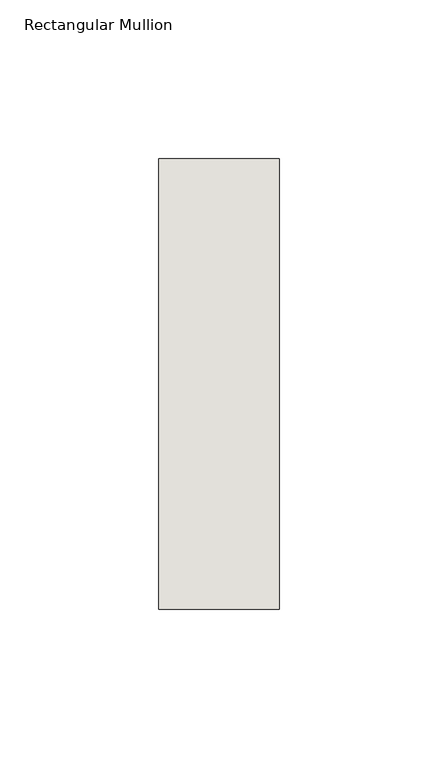
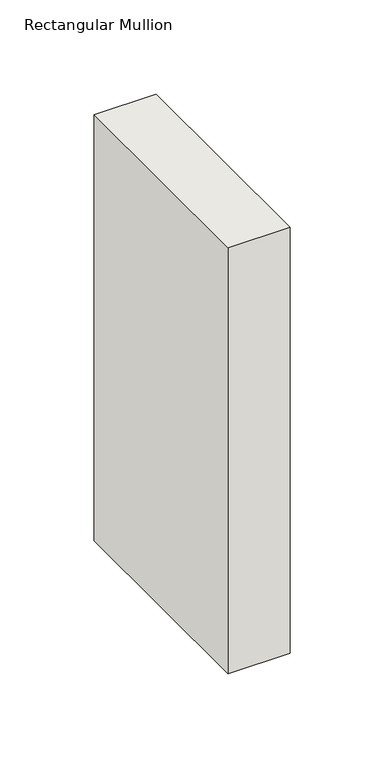
"""IFC4 building model written with IfcOpenShell, lengths in millimetres: wall geometry, Rectangular Mullion : NLRS_21_CWM_hsb-regel 38x142_gen_rsf."""

import ifcopenshell
import ifcopenshell.guid

model = None  # the IFC model being written
_history = None  # IfcOwnerHistory: only IFC2X3 demands one
_inside = {}  # id of a spatial element -> (the spatial element, [elements in it])
_under = {}  # id of a project, library or spatial element -> (it, [spatial elements below it])
_declared = {}  # id of a project -> (the project, [libraries it declares])
_typed = {}  # id of a type object -> (the type object, [elements of that type])
_made_of = {}  # id of a material, layer set ... -> (it, [elements and type objects made of it])


def new_model(schema):
    """Start an empty IFC model of exactly this schema.

    Asked for "IFC4X3", IfcOpenShell would pick the latest addendum, in which some entities
    have other attributes; the version numbers below select the first issue.
    IFC2X3 requires an IfcOwnerHistory on every rooted entity: one is made here for all.
    """
    global model, _history
    if schema == "IFC4X3":
        model = ifcopenshell.file(schema_version=(4, 3, 0, 0))
    else:
        model = ifcopenshell.file(schema=schema)
    _inside.clear()
    _under.clear()
    _declared.clear()
    _typed.clear()
    _made_of.clear()
    _history = None
    if model.schema == "IFC2X3":
        org = make("IfcOrganization", Name="unknown")
        user = make(
            "IfcPersonAndOrganization",
            ThePerson=make("IfcPerson", FamilyName="unknown"),
            TheOrganization=org,
        )
        app = make(
            "IfcApplication",
            ApplicationDeveloper=org,
            Version="unknown",
            ApplicationFullName="unknown",
            ApplicationIdentifier="unknown",
        )
        _history = make(
            "IfcOwnerHistory",
            OwningUser=user,
            OwningApplication=app,
            ChangeAction="ADDED",
            CreationDate=0,
        )
    return model


def make(cls, **values):
    """One entity of the class cls with the attributes given. An attribute that is None is left unset."""
    return model.create_entity(
        cls, **{name: value for name, value in values.items() if value is not None}
    )


def rooted(cls, **values):
    """An entity with a GlobalId (a new one), such as an element, a storey or a relation."""
    return make(cls, GlobalId=ifcopenshell.guid.new(), OwnerHistory=_history, **values)


def si_unit(unit_type, name, prefix=None):
    """IfcSIUnit, for example si_unit("LENGTHUNIT", "METRE", prefix="MILLI")."""
    return make("IfcSIUnit", UnitType=unit_type, Prefix=prefix, Name=name)


def assignment(units):
    """IfcUnitAssignment: the units of a project."""
    return None if units is None else make("IfcUnitAssignment", Units=units)


def point(xyz):
    """IfcCartesianPoint."""
    return None if xyz is None else make("IfcCartesianPoint", Coordinates=xyz)


def direction(xyz):
    """IfcDirection."""
    return None if xyz is None else make("IfcDirection", DirectionRatios=xyz)


def frame(location, z_axis=None, x_axis=None):
    """IfcAxis2Placement3D, a coordinate frame: its origin and axes. An axis left out is left unset."""
    return make(
        "IfcAxis2Placement3D",
        Location=point(location),
        Axis=direction(z_axis),
        RefDirection=direction(x_axis),
    )


def origin():
    """The frame at (0, 0, 0) with its axes left unset."""
    return frame((0.0, 0.0, 0.0))


def place(relative_to, where):
    """IfcLocalPlacement: puts the frame where relative to a parent placement (None: the world)."""
    return make(
        "IfcLocalPlacement", PlacementRelTo=relative_to, RelativePlacement=where
    )


def context(
    kind, dimensions, precision=None, world=None, true_north=None, identifier=None
):
    """IfcGeometricRepresentationContext, for example the 3D "Model" context."""
    return make(
        "IfcGeometricRepresentationContext",
        ContextIdentifier=identifier,
        ContextType=kind,
        CoordinateSpaceDimension=dimensions,
        Precision=precision,
        WorldCoordinateSystem=world,
        TrueNorth=true_north,
    )


def project(units=None, contexts=None):
    """IfcProject with its units and contexts."""
    return rooted(
        "IfcProject",
        Name="project",
        RepresentationContexts=contexts,
        UnitsInContext=assignment(units),
    )


def spatial(cls, under=None, at=None, **own):
    """A site, building, storey or space (cls), placed at a placement, below another one or the project."""
    s = rooted(cls, ObjectPlacement=at, **own)
    if under is not None:
        _under.setdefault(under.id(), (under, []))[1].append(s)
    return s


def polyline(points):
    """IfcPolyline through the points."""
    return make("IfcPolyline", Points=[point(p) for p in points])


def outline(outer, holes=None, kind="AREA"):
    """IfcArbitraryClosedProfileDef: a profile drawn as a closed curve; with holes, ...WithVoids."""
    if holes is None:
        return make("IfcArbitraryClosedProfileDef", ProfileType=kind, OuterCurve=outer)
    return make(
        "IfcArbitraryProfileDefWithVoids",
        ProfileType=kind,
        OuterCurve=outer,
        InnerCurves=holes,
    )


def extrude(swept, where, along, depth):
    """IfcExtrudedAreaSolid: the profile swept, set in the frame where, extruded along a direction by depth."""
    return make(
        "IfcExtrudedAreaSolid",
        SweptArea=swept,
        Position=where,
        ExtrudedDirection=direction(along),
        Depth=depth,
    )


def shape(context_of_items, identifier, shape_type, items):
    """IfcShapeRepresentation: the items that make up one representation, for example the "Body"."""
    return make(
        "IfcShapeRepresentation",
        ContextOfItems=context_of_items,
        RepresentationIdentifier=identifier,
        RepresentationType=shape_type,
        Items=items,
    )


def source(mapping_origin, context_of_items, identifier, shape_type, items):
    """IfcRepresentationMap: a shape defined once, which mapped items show again and again."""
    return make(
        "IfcRepresentationMap",
        MappingOrigin=mapping_origin,
        MappedRepresentation=shape(context_of_items, identifier, shape_type, items),
    )


def transform(
    local_origin,
    x_axis=None,
    y_axis=None,
    z_axis=None,
    scale=None,
    scale2=None,
    scale3=None,
    uniform=True,
):
    """IfcCartesianTransformationOperator3D, or its non-uniform kind. x_axis, y_axis, z_axis: its Axis1, 2, 3."""
    if uniform:
        return make(
            "IfcCartesianTransformationOperator3D",
            Axis1=direction(x_axis),
            Axis2=direction(y_axis),
            LocalOrigin=point(local_origin),
            Scale=scale,
            Axis3=direction(z_axis),
        )
    return make(
        "IfcCartesianTransformationOperator3DnonUniform",
        Axis1=direction(x_axis),
        Axis2=direction(y_axis),
        LocalOrigin=point(local_origin),
        Scale=scale,
        Axis3=direction(z_axis),
        Scale2=scale2,
        Scale3=scale3,
    )


def mapped(mapping_source, mapping_target):
    """IfcMappedItem: shows the shape of a source again, moved by a transform."""
    return make(
        "IfcMappedItem", MappingSource=mapping_source, MappingTarget=mapping_target
    )


def made_of(thing, what):
    """Note that an element or type object is made of a material, layer set ...; save() writes the relation."""
    if what is not None:
        _made_of.setdefault(what.id(), (what, []))[1].append(thing)
    return thing


def element(
    cls,
    number,
    at=None,
    inside=None,
    cuts=None,
    type_object=None,
    material=None,
    context=None,
    identifier="Body",
    shape_type=None,
    held_by="IfcProductDefinitionShape",
    body=None,
    shapes=None,
    **own,
):
    """One element of the class cls, such as IfcWall. Its Tag is "e" and its number.

    at: its placement. inside: the storey or other place that contains it. cuts: it is an
    opening in that element (IfcRelVoidsElement). A single representation is given by context,
    identifier, shape_type and body (its items); several are given by shapes. held_by: the class
    of the entity that holds the representations. save() writes the other relations.
    """
    e = rooted(cls, Tag="e%d" % number, ObjectPlacement=at, **own)
    if body is not None:
        shapes = [shape(context, identifier, shape_type, body)]
    if shapes is not None:
        e.Representation = make(held_by, Representations=shapes)
    if inside is not None:
        _inside.setdefault(inside.id(), (inside, []))[1].append(e)
    if cuts is not None:
        rooted(
            "IfcRelVoidsElement", RelatingBuildingElement=cuts, RelatedOpeningElement=e
        )
    if type_object is not None:
        _typed.setdefault(type_object.id(), (type_object, []))[1].append(e)
    return made_of(e, material)


def aggregate(whole, parts):
    """IfcRelAggregates: a whole, such as a stair, and the parts it consists of."""
    return rooted("IfcRelAggregates", RelatingObject=whole, RelatedObjects=parts)


def save(model, path):
    """Write the relations noted so far, then the file.

    IfcRelAggregates (storeys below a building ...), IfcRelContainedInSpatialStructure (elements
    in a storey), IfcRelDefinesByType, IfcRelAssociatesMaterial and IfcRelDeclares: one each for
    every whole, place, type object, material and project.
    """
    for whole, parts in _under.values():
        aggregate(whole, parts)
    for where, things in _inside.values():
        rooted(
            "IfcRelContainedInSpatialStructure",
            RelatedElements=things,
            RelatingStructure=where,
        )
    for kind, things in _typed.values():
        rooted("IfcRelDefinesByType", RelatedObjects=things, RelatingType=kind)
    for what, things in _made_of.values():
        rooted("IfcRelAssociatesMaterial", RelatedObjects=things, RelatingMaterial=what)
    for by, libraries in _declared.values():
        rooted("IfcRelDeclares", RelatingContext=by, RelatedDefinitions=libraries)
    model.write(path)


def rectangular_mullion_f581aa4a(model_context):
    return source(origin(), model_context, "Body", "SweptSolid", [
        extrude(outline(polyline([(19.0, -71.0), (-19.0, -71.0), (-19.0, 71.0), (19.0, 71.0), (19.0, -71.0)])), frame((0.0, 0.0, -276.0), z_axis=(0.0, 0.0, 1.0), x_axis=(1.0, 0.0, 0.0)), (0.0, 0.0, 1.0), 276.0),
    ])


if __name__ == "__main__":
    model = new_model("IFC4")
    model_context = context("Model", 3, world=origin())
    ifc_project = project(units=[si_unit("LENGTHUNIT", "METRE", prefix="MILLI")], contexts=[model_context])
    site = spatial("IfcSite", under=ifc_project)
    building = spatial("IfcBuilding", under=site)
    placement = place(None, origin())
    rectangular_mullion_shape = rectangular_mullion_f581aa4a(model_context)
    element("IfcWall", 1, ObjectType="Rectangular Mullion : NLRS_21_CWM_hsb-regel 38x142_gen_rsf", at=placement, inside=building, context=model_context, shape_type="MappedRepresentation", body=[
        mapped(rectangular_mullion_shape, transform((0.0, 0.0, 0.0), x_axis=(1.0, 0.0, 0.0), y_axis=(0.0, 1.0, 0.0), z_axis=(0.0, 0.0, 1.0))),
    ])
    save(model, "model.ifc")

# Revit data of these elements
# Type "Rectangular Mullion : NLRS_21_CWM_hsb-regel 38x142_gen_rsf"
#   Type IfcGUID = "07M7mRoiH1CR8m_RSKIwpF"
#   Assembly Code = "21.10"
#   IfcExportAs = "IfcWall"
#   built-in parameter 1007322 = 0.465879 (stored number, unit not read)
#   built-in parameter 1007321 = 0.062336 (stored number, unit not read)
#   built-in parameter 1007320 = 0.062336 (stored number, unit not read)
# Element 1 (IfcWall, "Rectangular Mullion : NLRS_21_CWM_hsb-regel 38x142_gen_rsf")
#   Materials on its faces: "NLRS_i2_hout naaldhout vuren_gen_rsf"
# Materials
#   "NLRS_i2_hout naaldhout vuren_gen_rsf": class "I - Hout", colour RGB 234 199 147, transparency 0, Keynote = "i2", Manufacturer = "Revit Standards Foundation", URL = "www.revitstandards.org", Description = "hout vuren", Cost = 0
